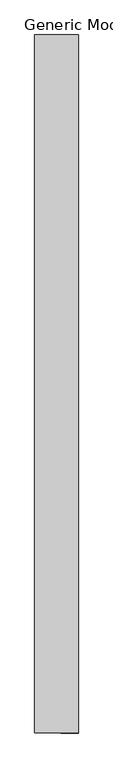
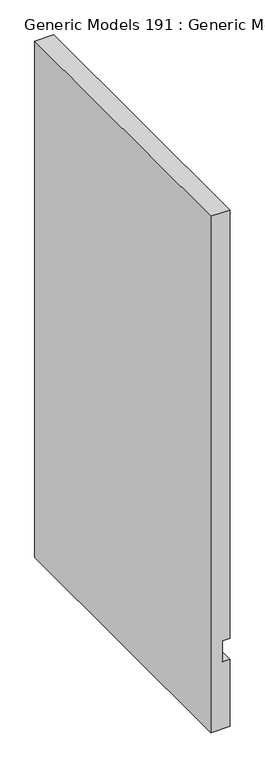
"""IFC4 building model written with IfcOpenShell, lengths in millimetres: proxy geometry, Generic Models 191 : Generic Models 1."""

from ifc_helpers import new_model, si_unit, frame, origin, place, context, project, spatial, polyline, outline, extrude, source, transform, mapped, element, save


def generic_models_191_generic_models_1_c7679766(model_context):
    return source(origin(), model_context, "Body", "SweptSolid", [
        extrude(outline(polyline([(-1916.5098206, 50127.9071108), (-1916.5098206, 50204.1071108), (-1633.3277575, 50204.1071108), (-1633.3277575, 50173.9446108), (-1544.4277575, 50173.9446108), (-1544.4277575, 50204.1071108), (263.7731772, 50204.1071108), (263.7731772, 50127.9071108), (-1916.5098206, 50127.9071108)])), frame((0.0, 0.0, 0.0), z_axis=(0.0, 1.0, 0.0), x_axis=(0.0, 0.0, 1.0)), (0.0, 0.0, 1.0), 1219.2),
    ])


if __name__ == "__main__":
    model = new_model("IFC4")
    model_context = context("Model", 3, world=origin())
    ifc_project = project(units=[si_unit("LENGTHUNIT", "METRE", prefix="MILLI")], contexts=[model_context])
    site = spatial("IfcSite", under=ifc_project)
    building = spatial("IfcBuilding", under=site)
    placement = place(None, origin())
    generic_models_191_generic_models_1_shape = generic_models_191_generic_models_1_c7679766(model_context)
    element("IfcBuildingElementProxy", 1, Name="Generic Models 191 : Generic Models 1", ObjectType="Generic Models 191 : Generic Models 1", at=placement, inside=building, context=model_context, shape_type="MappedRepresentation", body=[
        mapped(generic_models_191_generic_models_1_shape, transform((0.0, 0.0, 0.0), x_axis=(1.0, 0.0, 0.0), y_axis=(0.0, 1.0, 0.0), z_axis=(0.0, 0.0, 1.0))),
    ])
    save(model, "model.ifc")

# Revit data of these elements
# Element 1 (IfcBuildingElementProxy, "Generic Models 191 : Generic Models 1")
#   Materials on its faces: "(S) SOUND BATT. INSULATION (THICKNESS TO MATCH WALL DEPTH)"
# Materials
#   "(S) SOUND BATT. INSULATION (THICKNESS TO MATCH WALL DEPTH)": class "Unassigned", colour RGB 255 255 255, transparency 0, Cost = 0
